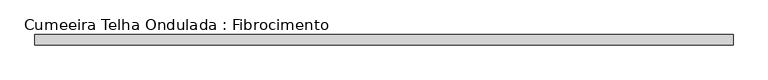
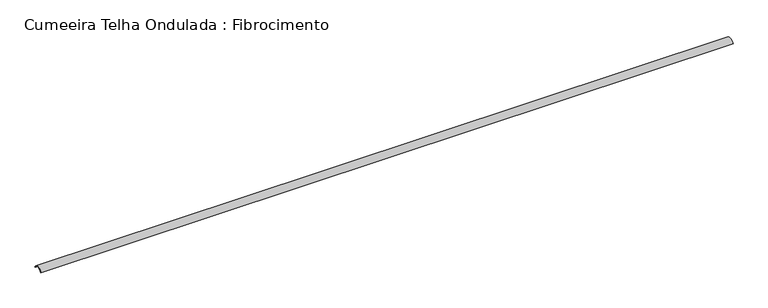
"""IFC4 building model written with IfcOpenShell, lengths in millimetres: beam geometry, Cumeeira Telha Ondulada : Fibrocimento."""

from ifc_helpers import new_model, si_unit, point, frame, frame_2d, origin, place, context, project, spatial, polyline, circle_curve, trimmed, segment, composite_curve, outline, extrude, source, transform, mapped, element, save


def cumeeira_telha_ondulada_fibrocimento_a8dbf5af(model_context):
    return source(origin(), model_context, "Body", "SweptSolid", [
        extrude(outline(composite_curve([segment(polyline([(58.3970135, 42.4437972), (53.9055884, 40.2467307)]), True, "CONTINUOUS"), segment(trimmed(circle_curve(frame_2d((-1.6029865, 13.0936483)), 61.7939461), [point((53.9055884, 40.2467307))], [point((-57.1115615, 40.2467307))], True, "CARTESIAN"), True, "CONTINUOUS"), segment(polyline([(-57.1115615, 40.2467307), (-61.6029865, 42.4437972)]), True, "CONTINUOUS"), segment(trimmed(circle_curve(frame_2d((-1.6029865, 13.0936483)), 66.7939461), [point((-61.6029865, 42.4437972))], [point((58.3970135, 42.4437972))], False, "CARTESIAN"), True, "CONTINUOUS")], self_intersect=False)), frame((-3970.0, 0.0, 0.0), z_axis=(1.0, 0.0, 0.0), x_axis=(0.0, 1.0, 0.0)), (0.0, 0.0, 1.0), 7940.0),
    ])


if __name__ == "__main__":
    model = new_model("IFC4")
    model_context = context("Model", 3, world=origin())
    ifc_project = project(units=[si_unit("LENGTHUNIT", "METRE", prefix="MILLI")], contexts=[model_context])
    site = spatial("IfcSite", under=ifc_project)
    building = spatial("IfcBuilding", under=site)
    placement = place(None, origin())
    cumeeira_telha_ondulada_fibrocimento_shape = cumeeira_telha_ondulada_fibrocimento_a8dbf5af(model_context)
    element("IfcBeam", 1, ObjectType="Cumeeira Telha Ondulada : Fibrocimento", at=placement, inside=building, context=model_context, shape_type="MappedRepresentation", body=[
        mapped(cumeeira_telha_ondulada_fibrocimento_shape, transform((0.0, 0.0, 0.0), x_axis=(1.0, 0.0, 0.0), y_axis=(0.0, 1.0, 0.0), z_axis=(0.0, 0.0, 1.0))),
    ])
    save(model, "model.ifc")

# Revit data of these elements
# Type "Cumeeira Telha Ondulada : Fibrocimento"
#   Cost = 5
#   Length [instance default] = 1.524 m
#   b = 0.07 m
#   h = 0.16 m
#   Structural Material = .TELHA DE FIBROCIMENTO
#   Assembly Code = ""
# Element 1 (IfcBeam, "Cumeeira Telha Ondulada : Fibrocimento")
#   Materials on its faces: ".TELHA DE FIBROCIMENTO"
# Materials
#   ".TELHA DE FIBROCIMENTO": class "CC_TELHADO", colour RGB 77 77 76, transparency 0, Description = "TELHA ONDULADA FIBROCIMENTO", Cost = 0
